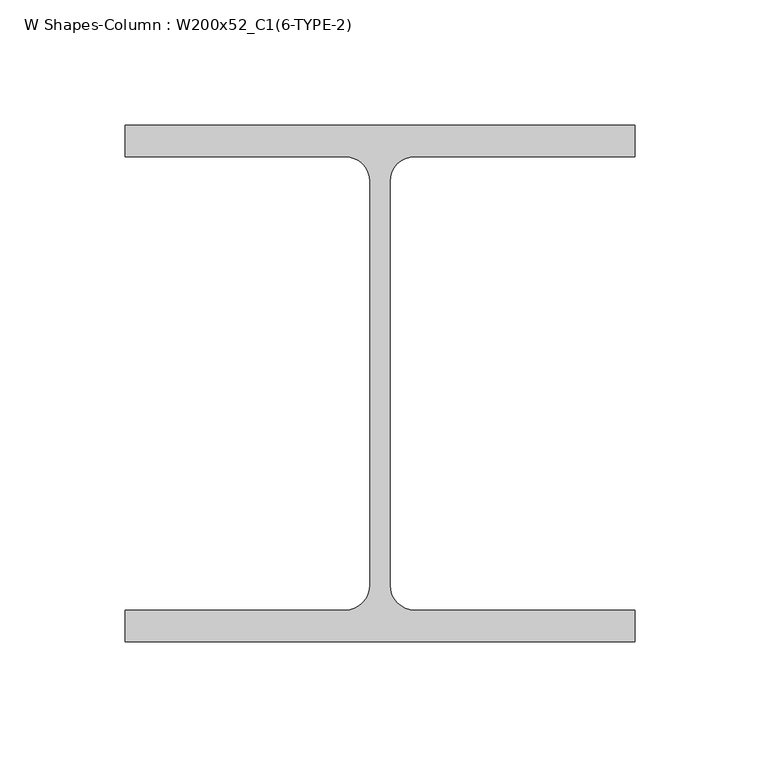
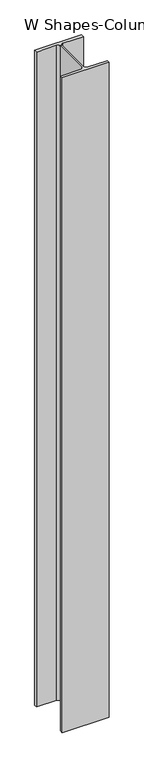
"""IFC4 building model written with IfcOpenShell, lengths in millimetres: column geometry, W Shapes-Column : W200x52_C1(6-TYPE-2)."""

from ifc_helpers import new_model, si_unit, point, frame, frame_2d, origin, place, context, project, spatial, polyline, circle_curve, trimmed, segment, composite_curve, outline, extrude, source, transform, mapped, element, save


def w_shapes_column_w200x52_c1_6_type_2_040e5d3a(model_context):
    return source(origin(), model_context, "Body", "SweptSolid", [
        extrude(outline(composite_curve([segment(polyline([(101.854, 103.124), (101.854, 90.551), (13.9446, 90.551)]), True, "CONTINUOUS"), segment(trimmed(circle_curve(frame_2d((13.9446, 80.5434)), 10.0076), [point((13.9446, 90.551))], [point((3.937, 80.5434))], True, "CARTESIAN"), True, "CONTINUOUS"), segment(polyline([(3.937, 80.5434), (3.937, -80.5434)]), True, "CONTINUOUS"), segment(trimmed(circle_curve(frame_2d((13.9446, -80.5434)), 10.0076), [point((3.937, -80.5434))], [point((13.9446, -90.551))], True, "CARTESIAN"), True, "CONTINUOUS"), segment(polyline([(13.9446, -90.551), (101.854, -90.551), (101.854, -103.124), (-101.854, -103.124), (-101.854, -90.551), (-13.9446, -90.551)]), True, "CONTINUOUS"), segment(trimmed(circle_curve(frame_2d((-13.9446, -80.5434)), 10.0076), [point((-13.9446, -90.551))], [point((-3.937, -80.5434))], True, "CARTESIAN"), True, "CONTINUOUS"), segment(polyline([(-3.937, -80.5434), (-3.937, 80.5434)]), True, "CONTINUOUS"), segment(trimmed(circle_curve(frame_2d((-13.9446, 80.5434)), 10.0076), [point((-3.937, 80.5434))], [point((-13.9446, 90.551))], True, "CARTESIAN"), True, "CONTINUOUS"), segment(polyline([(-13.9446, 90.551), (-101.854, 90.551), (-101.854, 103.124), (101.854, 103.124)]), True, "CONTINUOUS")], self_intersect=False)), frame((0.0, 0.0, 3220.0), z_axis=(0.0, 0.0, 1.0), x_axis=(1.0, 0.0, 0.0)), (0.0, 0.0, 1.0), 3000.0),
    ])


if __name__ == "__main__":
    model = new_model("IFC4")
    model_context = context("Model", 3, world=origin())
    ifc_project = project(units=[si_unit("LENGTHUNIT", "METRE", prefix="MILLI")], contexts=[model_context])
    site = spatial("IfcSite", under=ifc_project)
    building = spatial("IfcBuilding", under=site)
    placement = place(None, origin())
    w_shapes_column_w200x52_c1_6_type_2_shape = w_shapes_column_w200x52_c1_6_type_2_040e5d3a(model_context)
    element("IfcColumn", 1, ObjectType="W Shapes-Column : W200x52_C1(6-TYPE-2)", at=placement, inside=building, context=model_context, shape_type="MappedRepresentation", body=[
        mapped(w_shapes_column_w200x52_c1_6_type_2_shape, transform((0.0, 0.0, 0.0), x_axis=(1.0, 0.0, 0.0), y_axis=(0.0, 1.0, 0.0), z_axis=(0.0, 0.0, 1.0))),
    ])
    save(model, "model.ifc")

# Revit data of these elements
# Type "W Shapes-Column : W200x52_C1(6-TYPE-2)"
#   Section Name Key = "W8X35"
#   Assembly Code = "B10"
#   Width = 20.3708 cm
#   Web Thickness = 0.7874 cm
#   Web Fillet = 1.0008 cm
#   Warping Constant = 166223.7 cm⁶
#   Torsional Moment of Inertia = 32.0082 cm⁴
#   Section Area = 66.4515 cm²
#   Plastic Modulus weak axis = 263.832 cm³
#   Plastic Modulus strong axis = 568.631 cm³
#   Perimeter = 1.1936 m²/m
#   Nominal Weight = 52.0857 kgf/m
#   Moment of Inertia weak axis = 1773.15 cm⁴
#   Moment of Inertia strong axis = 5286.14 cm⁴
#   Height = 20.6248 cm
#   Flange Thickness = 1.2573 cm
#   Elastic Modulus weak axis = 173.703 cm³
#   Elastic Modulus strong axis = 511.276 cm³
#   Clear Web Height = 14.605 cm
#   Centroid Vertical = 10.3124 cm
#   Centroid Horizontal = 10.1854 cm
#   Bolt Spacing = 13.97 cm
#   Structural Material [instance default] = Steel ASTM A992
#   Principal Axes Angle = 0
# Element 1 (IfcColumn, "W Shapes-Column : W200x52_C1(6-TYPE-2)")
#   Structural Material = none
# Materials
#   "Steel ASTM A992": class "Metal", colour RGB 199 199 199, transparency 0, Description = "Structural steel 50ksi", Cost = 0
